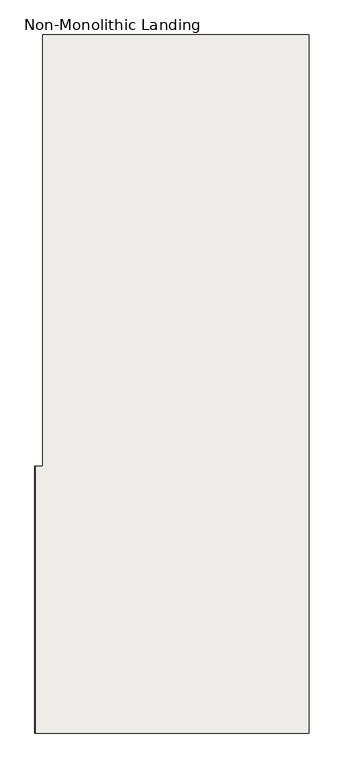
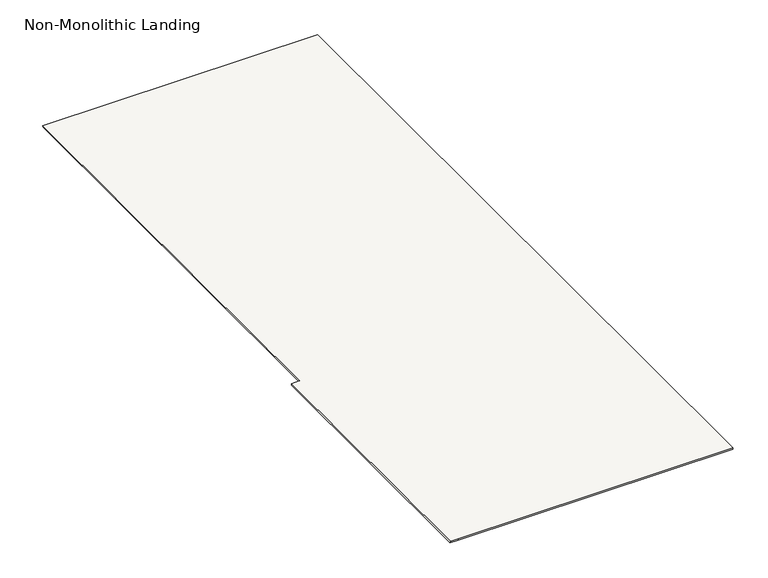
"""IFC4 building model written with IfcOpenShell, lengths in millimetres: slab geometry, Non-Monolithic Landing."""

from ifc_helpers import new_model, si_unit, origin, place, context, project, spatial, faceted_brep, source, transform, mapped, element, save


def non_monolithic_landing_ebe2e398(model_context):
    return source(origin(), model_context, "Body", "Brep", [
        faceted_brep([(-13356.0599092, 11395.4345331, 24235.2941176), (-13356.9099092, 11395.4345331, 24229.2941176), (-13356.9099092, 10295.4345331, 24229.2941176), (-13356.0599092, 10295.4345331, 24235.2941176), (-13325.0, 12075.4345331, 24235.2941176), (-13325.0, 11395.4345331, 24235.2941176), (-13325.0, 10295.4345331, 24235.2941176), (-12225.0, 10295.4345331, 24235.2941176), (-12225.0, 13175.4345331, 24235.2941176), (-13325.0, 13175.4345331, 24235.2941176), (-13325.0, 11395.4345331, 24229.2941176), (-13325.0, 12075.4345331, 24229.2941176), (-13324.15, 12075.4345331, 24229.2941176), (-13324.15, 13175.4345331, 24229.2941176), (-12225.0, 13175.4345331, 24229.2941176), (-12225.0, 10295.4345331, 24229.2941176), (-13325.0, 10295.4345331, 24229.2941176)], [[[0, 1, 2, 3]], [[4, 5, 0, 3, 6, 7, 8, 9]], [[10, 11, 12, 13, 14, 15, 16, 2, 1]], [[5, 4, 11, 10]], [[0, 5, 10, 1]], [[6, 3, 2, 16]], [[7, 6, 16, 15]], [[8, 7, 15, 14]], [[9, 8, 14, 13]], [[4, 12, 11]], [[12, 4, 9, 13]]]),
    ])


if __name__ == "__main__":
    model = new_model("IFC4")
    model_context = context("Model", 3, world=origin())
    ifc_project = project(units=[si_unit("LENGTHUNIT", "METRE", prefix="MILLI")], contexts=[model_context])
    site = spatial("IfcSite", under=ifc_project)
    building = spatial("IfcBuilding", under=site)
    placement = place(None, origin())
    non_monolithic_landing_shape = non_monolithic_landing_ebe2e398(model_context)
    element("IfcSlab", 1, ObjectType="Non-Monolithic Landing", at=placement, inside=building, context=model_context, shape_type="MappedRepresentation", body=[
        mapped(non_monolithic_landing_shape, transform((0.0, 0.0, 0.0), x_axis=(1.0, 0.0, 0.0), y_axis=(0.0, 1.0, 0.0), z_axis=(0.0, 0.0, 1.0))),
    ])
    save(model, "model.ifc")

# Revit data of these elements
# Element 1 (IfcSlab, "Non-Monolithic Landing")
#   Materials on its faces: "Steel, Paint Finish, Dark Gray"
# Materials
#   "Steel, Paint Finish, Dark Gray": class "Metal", colour RGB 89 89 89, transparency 0, Description = "Steel, paint finish, dark gray, glossy", Cost = 0
